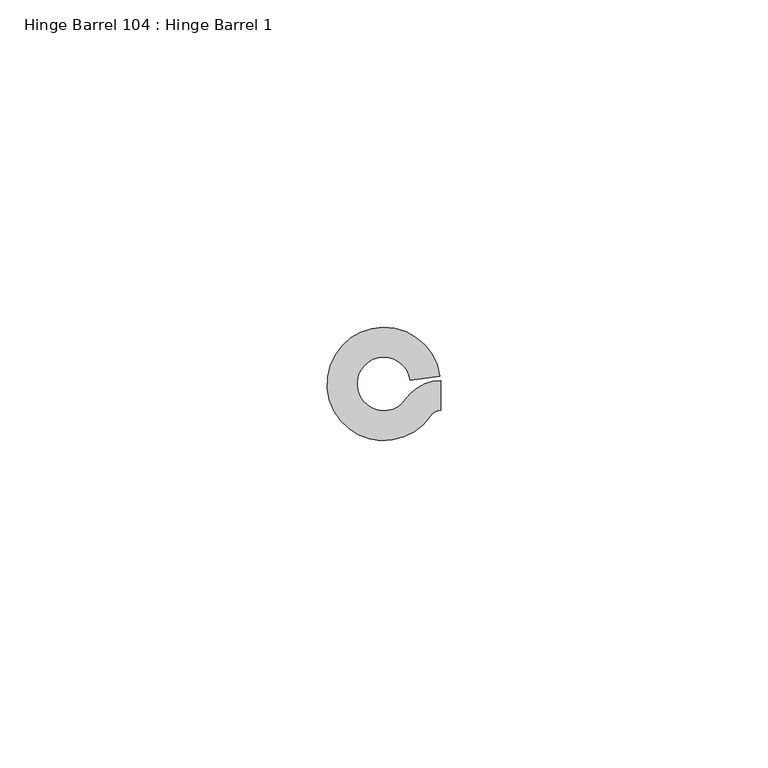
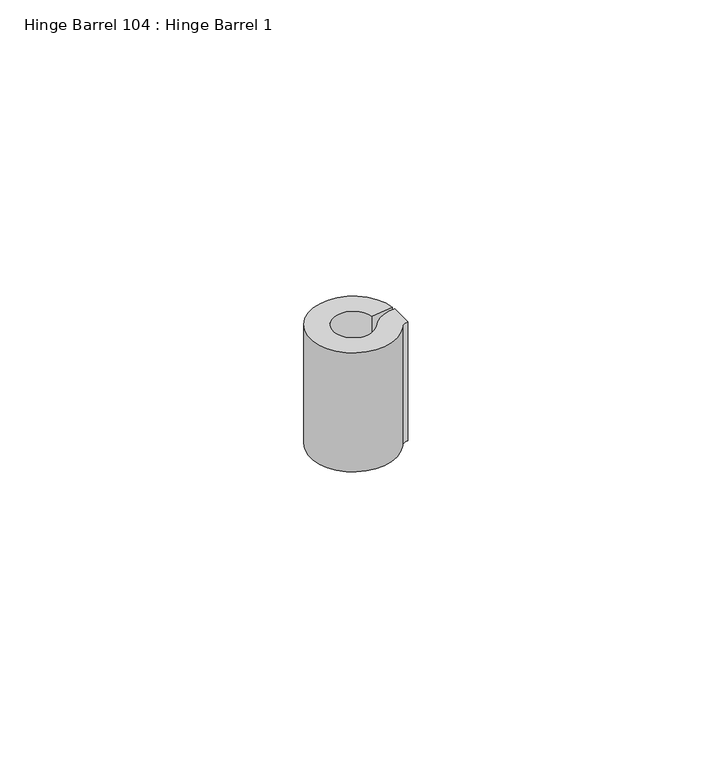
"""IFC4 building model written with IfcOpenShell, lengths in millimetres: proxy geometry, Hinge Barrel 104 : Hinge Barrel 1."""

from ifc_helpers import new_model, si_unit, point, frame, frame_2d, origin, place, context, project, spatial, polyline, circle_curve, trimmed, segment, composite_curve, outline, extrude, source, transform, mapped, element, save


def hinge_barrel_104_hinge_barrel_1_17cad03c(model_context):
    return source(origin(), model_context, "Body", "SweptSolid", [
        extrude(outline(composite_curve([segment(trimmed(circle_curve(frame_2d((587327.8245257, -533990.5568067)), 6.4044851), [point((587322.5194669, -533986.9688017))], [point((587327.8245257, -533984.1523216))], False, "CARTESIAN"), True, "CONTINUOUS"), segment(polyline([(587327.8245257, -533984.1523216), (587327.8245257, -533988.7163841)]), True, "CONTINUOUS"), segment(trimmed(circle_curve(frame_2d((587327.8245257, -533990.5568067)), 1.8404226), [point((587327.8245257, -533988.7163841))], [point((587326.3000393, -533989.5257409))], True, "CARTESIAN"), True, "CONTINUOUS"), segment(trimmed(circle_curve(frame_2d((587319.1320739, -533984.6777841)), 8.6534625), [point((587326.3000393, -533989.5257409))], [point((587327.7022899, -533983.4803654))], False, "CARTESIAN"), True, "CONTINUOUS"), segment(polyline([(587327.7022899, -533983.4803654), (587323.1821338, -533984.1119153)]), True, "CONTINUOUS"), segment(trimmed(circle_curve(frame_2d((587319.1320739, -533984.6777841)), 4.0894), [point((587323.1821338, -533984.1119153))], [point((587322.5194669, -533986.9688017))], True, "CARTESIAN"), True, "CONTINUOUS")], self_intersect=False)), frame((0.0, 0.0, 1149.35), z_axis=(0.0, 0.0, 1.0), x_axis=(1.0, 0.0, 0.0)), (0.0, 0.0, 1.0), 25.4),
    ])


if __name__ == "__main__":
    model = new_model("IFC4")
    model_context = context("Model", 3, world=origin())
    ifc_project = project(units=[si_unit("LENGTHUNIT", "METRE", prefix="MILLI")], contexts=[model_context])
    site = spatial("IfcSite", under=ifc_project)
    building = spatial("IfcBuilding", under=site)
    placement = place(None, origin())
    hinge_barrel_104_hinge_barrel_1_shape = hinge_barrel_104_hinge_barrel_1_17cad03c(model_context)
    element("IfcBuildingElementProxy", 1, Name="Hinge Barrel 104 : Hinge Barrel 1", ObjectType="Hinge Barrel 104 : Hinge Barrel 1", at=placement, inside=building, context=model_context, shape_type="MappedRepresentation", body=[
        mapped(hinge_barrel_104_hinge_barrel_1_shape, transform((0.0, 0.0, 0.0), x_axis=(1.0, 0.0, 0.0), y_axis=(0.0, 1.0, 0.0), z_axis=(0.0, 0.0, 1.0))),
    ])
    save(model, "model.ifc")

# Revit data of these elements
# Element 1 (IfcBuildingElementProxy, "Hinge Barrel 104 : Hinge Barrel 1")
#   Materials on its faces: "6\"X6\" WELD-ON STL BUTT HINGE"
# Materials
#   "6\"X6\" WELD-ON STL BUTT HINGE": class "Metal", colour RGB 189 187 185, transparency 0, Description = "Carbon steel", Cost = 0
